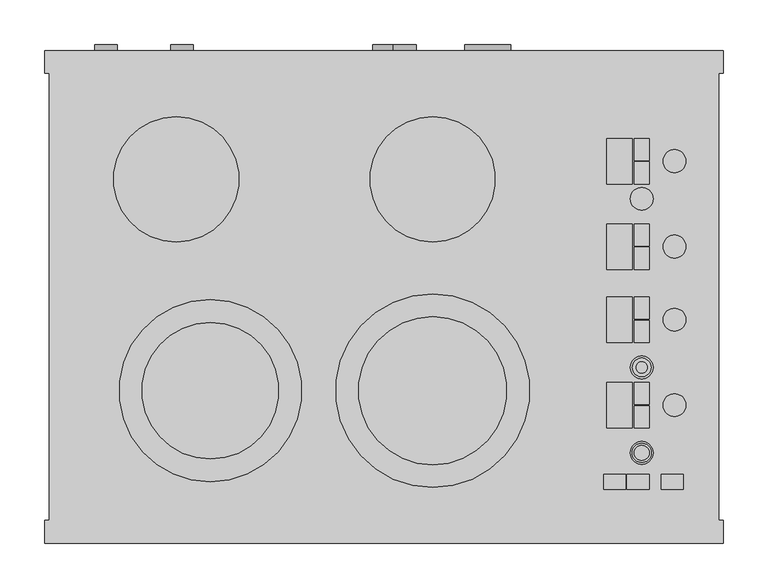
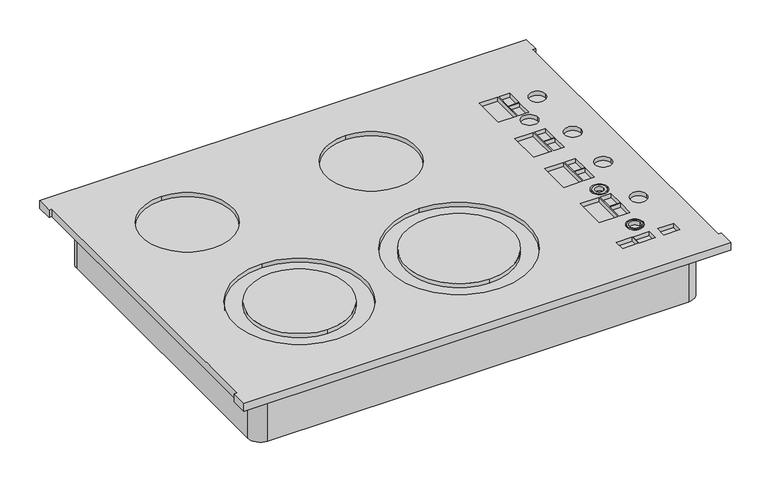
"""IFC4 building model written with IfcOpenShell, lengths in millimetres: proxy geometry, Cooktops_Electric_GE-Monogram_ZEU30RSFSS : Cooktops_Electric_GE-Monogram_ZEU30RSFSS."""

from ifc_helpers import new_model, si_unit, point, frame, frame_2d, origin, origin_with_axes, place, context, project, spatial, polyline, circle_curve, trimmed, segment, composite_curve, outline, extrude, source, transform, mapped, element, save


def specialty_equipment_065d487b(model_context):
    return source(origin(), model_context, "Body", "SweptSolid", [
        extrude(outline(composite_curve([segment(polyline([(-377.825, 274.6375), (377.825, 274.6375), (377.825, 249.2375), (373.215296, 249.2375), (373.215296, -249.2375), (377.825, -249.2375), (377.825, -274.6375)]), True, "CONTINUOUS"), segment(trimmed(circle_curve(frame_2d((0.0, 4104.744837)), 4395.65028), [point((377.825, -274.6375))], [point((-377.825, -274.6375))], False, "CARTESIAN"), True, "CONTINUOUS"), segment(polyline([(-377.825, -274.6375), (-377.825, -249.2375), (-373.215296, -249.2375), (-373.215296, 249.2375), (-377.825, 249.2375), (-377.825, 274.6375)]), True, "CONTINUOUS")], self_intersect=False), holes=[composite_curve([segment(trimmed(circle_curve(frame_2d((54.2006403, 131.1676685)), 69.85), [point((54.2006403, 201.0176685))], [point((54.2006403, 61.3176685))], True, "CARTESIAN"), True, "CONTINUOUS"), segment(trimmed(circle_curve(frame_2d((54.2006403, 131.1676685)), 69.85), [point((54.2006403, 61.3176685))], [point((54.2006403, 201.0176685))], True, "CARTESIAN"), True, "CONTINUOUS")], self_intersect=False), composite_curve([segment(trimmed(circle_curve(frame_2d((54.2006403, -104.6769785)), 107.95), [point((54.2006403, 3.2730215))], [point((54.2006403, -212.6269785))], True, "CARTESIAN"), True, "CONTINUOUS"), segment(trimmed(circle_curve(frame_2d((54.2006403, -104.6769785)), 107.95), [point((54.2006403, -212.6269785))], [point((54.2006403, 3.2730215))], True, "CARTESIAN"), True, "CONTINUOUS")], self_intersect=False), composite_curve([segment(trimmed(circle_curve(frame_2d((-193.4493597, -104.6769785)), 101.6), [point((-193.4493597, -3.0769785))], [point((-193.4493597, -206.2769785))], True, "CARTESIAN"), True, "CONTINUOUS"), segment(trimmed(circle_curve(frame_2d((-193.4493597, -104.6769785)), 101.6), [point((-193.4493597, -206.2769785))], [point((-193.4493597, -3.0769785))], True, "CARTESIAN"), True, "CONTINUOUS")], self_intersect=False), composite_curve([segment(trimmed(circle_curve(frame_2d((-231.5493597, 131.1676685)), 69.85), [point((-231.5493597, 201.0176685))], [point((-231.5493597, 61.3176685))], True, "CARTESIAN"), True, "CONTINUOUS"), segment(trimmed(circle_curve(frame_2d((-231.5493597, 131.1676685)), 69.85), [point((-231.5493597, 61.3176685))], [point((-231.5493597, 201.0176685))], True, "CARTESIAN"), True, "CONTINUOUS")], self_intersect=False), polyline([(276.5029806, 125.8458819), (276.5029806, 176.6458819), (247.9432042, 176.6458819), (247.9432042, 125.8458819), (276.5029806, 125.8458819)]), polyline([(295.3523984, 125.8458819), (295.3523984, 150.5447711), (278.8954782, 150.5447711), (278.8954782, 125.8458819), (295.3523984, 125.8458819)]), polyline([(295.3523984, 176.6458819), (278.8954782, 176.6458819), (278.8954782, 151.9469928), (295.3523984, 151.9469928), (295.3523984, 176.6458819)]), composite_curve([segment(trimmed(circle_curve(frame_2d((323.5654873, 151.2458819)), 12.7), [point((310.8654873, 151.2458819))], [point((336.2654873, 151.2458819))], True, "CARTESIAN"), True, "CONTINUOUS"), segment(trimmed(circle_curve(frame_2d((323.5654873, 151.2458819)), 12.7), [point((336.2654873, 151.2458819))], [point((310.8654873, 151.2458819))], True, "CARTESIAN"), True, "CONTINUOUS")], self_intersect=False), composite_curve([segment(trimmed(circle_curve(frame_2d((287.1239383, 109.3246752)), 12.7), [point((274.4239383, 109.3246752))], [point((299.8239383, 109.3246752))], True, "CARTESIAN"), True, "CONTINUOUS"), segment(trimmed(circle_curve(frame_2d((287.1239383, 109.3246752)), 12.7), [point((299.8239383, 109.3246752))], [point((274.4239383, 109.3246752))], True, "CARTESIAN"), True, "CONTINUOUS")], self_intersect=False), polyline([(276.5029806, 30.5958819), (276.5029806, 81.3958819), (247.9432042, 81.3958819), (247.9432042, 30.5958819), (276.5029806, 30.5958819)]), polyline([(295.3523984, 30.5958819), (295.3523984, 55.2947711), (278.8954782, 55.2947711), (278.8954782, 30.5958819), (295.3523984, 30.5958819)]), polyline([(295.3523984, 81.3958819), (278.8954782, 81.3958819), (278.8954782, 56.6969928), (295.3523984, 56.6969928), (295.3523984, 81.3958819)]), composite_curve([segment(trimmed(circle_curve(frame_2d((323.5654873, 55.9958819)), 12.7), [point((310.8654873, 55.9958819))], [point((336.2654873, 55.9958819))], True, "CARTESIAN"), True, "CONTINUOUS"), segment(trimmed(circle_curve(frame_2d((323.5654873, 55.9958819)), 12.7), [point((336.2654873, 55.9958819))], [point((310.8654873, 55.9958819))], True, "CARTESIAN"), True, "CONTINUOUS")], self_intersect=False), polyline([(276.5029806, -95.25), (247.9432042, -95.25), (247.9432042, -146.05), (276.5029806, -146.05), (276.5029806, -95.25)]), polyline([(295.3523984, -95.25), (278.8954782, -95.25), (278.8954782, -119.9488891), (295.3523984, -119.9488891), (295.3523984, -95.25)]), polyline([(295.3523984, -146.05), (295.3523984, -121.3511109), (278.8954782, -121.3511109), (278.8954782, -146.05), (295.3523984, -146.05)]), composite_curve([segment(trimmed(circle_curve(frame_2d((323.5654873, -120.65)), 12.7), [point((310.8654873, -120.65))], [point((336.2654873, -120.65))], True, "CARTESIAN"), True, "CONTINUOUS"), segment(trimmed(circle_curve(frame_2d((323.5654873, -120.65)), 12.7), [point((336.2654873, -120.65))], [point((310.8654873, -120.65))], True, "CARTESIAN"), True, "CONTINUOUS")], self_intersect=False), composite_curve([segment(trimmed(circle_curve(frame_2d((287.1239383, -78.7287933)), 12.7), [point((274.4239383, -78.7287933))], [point((299.8239383, -78.7287933))], True, "CARTESIAN"), True, "CONTINUOUS"), segment(trimmed(circle_curve(frame_2d((287.1239383, -78.7287933)), 12.7), [point((299.8239383, -78.7287933))], [point((274.4239383, -78.7287933))], True, "CARTESIAN"), True, "CONTINUOUS")], self_intersect=False), polyline([(276.5029806, 0.0), (247.9432042, 0.0), (247.9432042, -50.8), (276.5029806, -50.8), (276.5029806, 0.0)]), polyline([(295.3523984, 0.0), (278.8954782, 0.0), (278.8954782, -24.6988891), (295.3523984, -24.6988891), (295.3523984, 0.0)]), polyline([(295.3523984, -50.8), (295.3523984, -26.1011109), (278.8954782, -26.1011109), (278.8954782, -50.8), (295.3523984, -50.8)]), composite_curve([segment(trimmed(circle_curve(frame_2d((323.5654873, -25.4)), 12.7), [point((310.8654873, -25.4))], [point((336.2654873, -25.4))], True, "CARTESIAN"), True, "CONTINUOUS"), segment(trimmed(circle_curve(frame_2d((323.5654873, -25.4)), 12.7), [point((336.2654873, -25.4))], [point((310.8654873, -25.4))], True, "CARTESIAN"), True, "CONTINUOUS")], self_intersect=False), composite_curve([segment(trimmed(circle_curve(frame_2d((287.1239383, -173.9787933)), 12.7), [point((274.4239383, -173.9787933))], [point((299.8239383, -173.9787933))], True, "CARTESIAN"), True, "CONTINUOUS"), segment(trimmed(circle_curve(frame_2d((287.1239383, -173.9787933)), 12.7), [point((299.8239383, -173.9787933))], [point((274.4239383, -173.9787933))], True, "CARTESIAN"), True, "CONTINUOUS")], self_intersect=False), polyline([(295.3523984, -214.5130009), (295.3523984, -198.0560807), (270.6535092, -198.0560807), (270.6535092, -214.5130009), (295.3523984, -214.5130009)]), polyline([(244.5523984, -214.5130009), (269.2512875, -214.5130009), (269.2512875, -198.0560807), (244.5523984, -198.0560807), (244.5523984, -214.5130009)]), polyline([(333.4523984, -214.5130009), (333.4523984, -198.0560807), (308.7535092, -198.0560807), (308.7535092, -214.5130009), (333.4523984, -214.5130009)])]), frame((0.0, 0.0, 82.55), z_axis=(0.0, 0.0, 1.0), x_axis=(1.0, 0.0, 0.0)), (0.0, 0.0, 1.0), 12.7),
        extrude(outline(composite_curve([segment(trimmed(circle_curve(frame_2d((54.2006403, -104.6769785)), 82.55), [point((54.2006403, -22.1269785))], [point((54.2006403, -187.2269785))], False, "CARTESIAN"), True, "CONTINUOUS"), segment(trimmed(circle_curve(frame_2d((54.2006403, -104.6769785)), 82.55), [point((54.2006403, -187.2269785))], [point((54.2006403, -22.1269785))], False, "CARTESIAN"), True, "CONTINUOUS")], self_intersect=False)), frame((0.0, 0.0, 82.55), z_axis=(0.0, 0.0, 1.0), x_axis=(1.0, 0.0, 0.0)), (0.0, 0.0, 1.0), 12.7),
        extrude(outline(composite_curve([segment(trimmed(circle_curve(frame_2d((-193.4493597, -104.6769785)), 76.2), [point((-193.4493597, -28.4769785))], [point((-193.4493597, -180.8769785))], False, "CARTESIAN"), True, "CONTINUOUS"), segment(trimmed(circle_curve(frame_2d((-193.4493597, -104.6769785)), 76.2), [point((-193.4493597, -180.8769785))], [point((-193.4493597, -28.4769785))], False, "CARTESIAN"), True, "CONTINUOUS")], self_intersect=False)), frame((0.0, 0.0, 82.55), z_axis=(0.0, 0.0, 1.0), x_axis=(1.0, 0.0, 0.0)), (0.0, 0.0, 1.0), 12.7),
        extrude(outline(composite_curve([segment(trimmed(circle_curve(frame_2d((287.1239383, -173.9787933)), 10.7837612), [point((276.3401772, -173.9787933))], [point((297.9076995, -173.9787933))], False, "CARTESIAN"), True, "CONTINUOUS"), segment(trimmed(circle_curve(frame_2d((287.1239383, -173.9787933)), 10.7837612), [point((297.9076995, -173.9787933))], [point((276.3401772, -173.9787933))], False, "CARTESIAN"), True, "CONTINUOUS")], self_intersect=False), holes=[composite_curve([segment(trimmed(circle_curve(frame_2d((287.1239383, -173.9787933)), 8.3684562), [point((278.7554821, -173.9787933))], [point((295.4923945, -173.9787933))], True, "CARTESIAN"), True, "CONTINUOUS"), segment(trimmed(circle_curve(frame_2d((287.1239383, -173.9787933)), 8.3684562), [point((295.4923945, -173.9787933))], [point((278.7554821, -173.9787933))], True, "CARTESIAN"), True, "CONTINUOUS")], self_intersect=False)]), frame((0.0, 0.0, 82.55), z_axis=(0.0, 0.0, 1.0), x_axis=(1.0, 0.0, 0.0)), (0.0, 0.0, 1.0), 12.7),
        extrude(outline(composite_curve([segment(trimmed(circle_curve(frame_2d((287.1239383, -78.7287933)), 10.3621749), [point((276.7617634, -78.7287933))], [point((297.4861132, -78.7287933))], False, "CARTESIAN"), True, "CONTINUOUS"), segment(trimmed(circle_curve(frame_2d((287.1239383, -78.7287933)), 10.3621749), [point((297.4861132, -78.7287933))], [point((276.7617634, -78.7287933))], False, "CARTESIAN"), True, "CONTINUOUS")], self_intersect=False), holes=[composite_curve([segment(trimmed(circle_curve(frame_2d((287.1239383, -78.7287933)), 6.35), [point((280.7739383, -78.7287933))], [point((293.4739383, -78.7287933))], True, "CARTESIAN"), True, "CONTINUOUS"), segment(trimmed(circle_curve(frame_2d((287.1239383, -78.7287933)), 6.35), [point((293.4739383, -78.7287933))], [point((280.7739383, -78.7287933))], True, "CARTESIAN"), True, "CONTINUOUS")], self_intersect=False)]), frame((0.0, 0.0, 82.55), z_axis=(0.0, 0.0, 1.0), x_axis=(1.0, 0.0, 0.0)), (0.0, 0.0, 1.0), 12.7),
        extrude(outline(polyline([(276.5029806, 125.8458819), (247.9432042, 125.8458819), (247.9432042, 176.6458819), (276.5029806, 176.6458819), (276.5029806, 125.8458819)])), frame((0.0, 0.0, 82.55), z_axis=(0.0, 0.0, 1.0), x_axis=(1.0, 0.0, 0.0)), (0.0, 0.0, 1.0), 6.35),
        extrude(outline(polyline([(295.3523984, 125.8458819), (278.8954782, 125.8458819), (278.8954782, 150.5447711), (295.3523984, 150.5447711), (295.3523984, 125.8458819)])), frame((0.0, 0.0, 82.55), z_axis=(0.0, 0.0, 1.0), x_axis=(1.0, 0.0, 0.0)), (0.0, 0.0, 1.0), 6.35),
        extrude(outline(polyline([(295.3523984, 176.6458819), (295.3523984, 151.9469928), (278.8954782, 151.9469928), (278.8954782, 176.6458819), (295.3523984, 176.6458819)])), frame((0.0, 0.0, 82.55), z_axis=(0.0, 0.0, 1.0), x_axis=(1.0, 0.0, 0.0)), (0.0, 0.0, 1.0), 6.35),
        extrude(outline(composite_curve([segment(trimmed(circle_curve(frame_2d((323.5654873, 151.2458819)), 12.7), [point((310.8654873, 151.2458819))], [point((336.2654873, 151.2458819))], False, "CARTESIAN"), True, "CONTINUOUS"), segment(trimmed(circle_curve(frame_2d((323.5654873, 151.2458819)), 12.7), [point((336.2654873, 151.2458819))], [point((310.8654873, 151.2458819))], False, "CARTESIAN"), True, "CONTINUOUS")], self_intersect=False)), frame((0.0, 0.0, 82.55), z_axis=(0.0, 0.0, 1.0), x_axis=(1.0, 0.0, 0.0)), (0.0, 0.0, 1.0), 6.35),
        extrude(outline(composite_curve([segment(trimmed(circle_curve(frame_2d((287.1239383, 109.3246752)), 12.7), [point((274.4239383, 109.3246752))], [point((299.8239383, 109.3246752))], False, "CARTESIAN"), True, "CONTINUOUS"), segment(trimmed(circle_curve(frame_2d((287.1239383, 109.3246752)), 12.7), [point((299.8239383, 109.3246752))], [point((274.4239383, 109.3246752))], False, "CARTESIAN"), True, "CONTINUOUS")], self_intersect=False)), frame((0.0, 0.0, 82.55), z_axis=(0.0, 0.0, 1.0), x_axis=(1.0, 0.0, 0.0)), (0.0, 0.0, 1.0), 6.35),
        extrude(outline(polyline([(276.5029806, 30.5958819), (247.9432042, 30.5958819), (247.9432042, 81.3958819), (276.5029806, 81.3958819), (276.5029806, 30.5958819)])), frame((0.0, 0.0, 82.55), z_axis=(0.0, 0.0, 1.0), x_axis=(1.0, 0.0, 0.0)), (0.0, 0.0, 1.0), 6.35),
        extrude(outline(polyline([(295.3523984, 30.5958819), (278.8954782, 30.5958819), (278.8954782, 55.2947711), (295.3523984, 55.2947711), (295.3523984, 30.5958819)])), frame((0.0, 0.0, 82.55), z_axis=(0.0, 0.0, 1.0), x_axis=(1.0, 0.0, 0.0)), (0.0, 0.0, 1.0), 6.35),
        extrude(outline(polyline([(295.3523984, 81.3958819), (295.3523984, 56.6969928), (278.8954782, 56.6969928), (278.8954782, 81.3958819), (295.3523984, 81.3958819)])), frame((0.0, 0.0, 82.55), z_axis=(0.0, 0.0, 1.0), x_axis=(1.0, 0.0, 0.0)), (0.0, 0.0, 1.0), 6.35),
        extrude(outline(composite_curve([segment(trimmed(circle_curve(frame_2d((323.5654873, 55.9958819)), 12.7), [point((310.8654873, 55.9958819))], [point((336.2654873, 55.9958819))], False, "CARTESIAN"), True, "CONTINUOUS"), segment(trimmed(circle_curve(frame_2d((323.5654873, 55.9958819)), 12.7), [point((336.2654873, 55.9958819))], [point((310.8654873, 55.9958819))], False, "CARTESIAN"), True, "CONTINUOUS")], self_intersect=False)), frame((0.0, 0.0, 82.55), z_axis=(0.0, 0.0, 1.0), x_axis=(1.0, 0.0, 0.0)), (0.0, 0.0, 1.0), 6.35),
        extrude(outline(polyline([(276.5029806, -95.25), (276.5029806, -146.05), (247.9432042, -146.05), (247.9432042, -95.25), (276.5029806, -95.25)])), frame((0.0, 0.0, 82.55), z_axis=(0.0, 0.0, 1.0), x_axis=(1.0, 0.0, 0.0)), (0.0, 0.0, 1.0), 6.35),
        extrude(outline(polyline([(295.3523984, -95.25), (295.3523984, -119.9488891), (278.8954782, -119.9488891), (278.8954782, -95.25), (295.3523984, -95.25)])), frame((0.0, 0.0, 82.55), z_axis=(0.0, 0.0, 1.0), x_axis=(1.0, 0.0, 0.0)), (0.0, 0.0, 1.0), 6.35),
        extrude(outline(polyline([(295.3523984, -146.05), (278.8954782, -146.05), (278.8954782, -121.3511109), (295.3523984, -121.3511109), (295.3523984, -146.05)])), frame((0.0, 0.0, 82.55), z_axis=(0.0, 0.0, 1.0), x_axis=(1.0, 0.0, 0.0)), (0.0, 0.0, 1.0), 6.35),
        extrude(outline(composite_curve([segment(trimmed(circle_curve(frame_2d((323.5654873, -120.65)), 12.7), [point((310.8654873, -120.65))], [point((336.2654873, -120.65))], False, "CARTESIAN"), True, "CONTINUOUS"), segment(trimmed(circle_curve(frame_2d((323.5654873, -120.65)), 12.7), [point((336.2654873, -120.65))], [point((310.8654873, -120.65))], False, "CARTESIAN"), True, "CONTINUOUS")], self_intersect=False)), frame((0.0, 0.0, 82.55), z_axis=(0.0, 0.0, 1.0), x_axis=(1.0, 0.0, 0.0)), (0.0, 0.0, 1.0), 6.35),
        extrude(outline(composite_curve([segment(trimmed(circle_curve(frame_2d((287.1239383, -78.7287933)), 12.7), [point((274.4239383, -78.7287933))], [point((299.8239383, -78.7287933))], False, "CARTESIAN"), True, "CONTINUOUS"), segment(trimmed(circle_curve(frame_2d((287.1239383, -78.7287933)), 12.7), [point((299.8239383, -78.7287933))], [point((274.4239383, -78.7287933))], False, "CARTESIAN"), True, "CONTINUOUS")], self_intersect=False), holes=[composite_curve([segment(trimmed(circle_curve(frame_2d((287.1239383, -78.7287933)), 10.3621749), [point((276.7617634, -78.7287933))], [point((297.4861132, -78.7287933))], True, "CARTESIAN"), True, "CONTINUOUS"), segment(trimmed(circle_curve(frame_2d((287.1239383, -78.7287933)), 10.3621749), [point((297.4861132, -78.7287933))], [point((276.7617634, -78.7287933))], True, "CARTESIAN"), True, "CONTINUOUS")], self_intersect=False)]), frame((0.0, 0.0, 82.55), z_axis=(0.0, 0.0, 1.0), x_axis=(1.0, 0.0, 0.0)), (0.0, 0.0, 1.0), 6.35),
        extrude(outline(polyline([(276.5029806, 0.0), (276.5029806, -50.8), (247.9432042, -50.8), (247.9432042, 0.0), (276.5029806, 0.0)])), frame((0.0, 0.0, 82.55), z_axis=(0.0, 0.0, 1.0), x_axis=(1.0, 0.0, 0.0)), (0.0, 0.0, 1.0), 6.35),
        extrude(outline(polyline([(295.3523984, 0.0), (295.3523984, -24.6988891), (278.8954782, -24.6988891), (278.8954782, 0.0), (295.3523984, 0.0)])), frame((0.0, 0.0, 82.55), z_axis=(0.0, 0.0, 1.0), x_axis=(1.0, 0.0, 0.0)), (0.0, 0.0, 1.0), 6.35),
        extrude(outline(polyline([(295.3523984, -50.8), (278.8954782, -50.8), (278.8954782, -26.1011109), (295.3523984, -26.1011109), (295.3523984, -50.8)])), frame((0.0, 0.0, 82.55), z_axis=(0.0, 0.0, 1.0), x_axis=(1.0, 0.0, 0.0)), (0.0, 0.0, 1.0), 6.35),
        extrude(outline(composite_curve([segment(trimmed(circle_curve(frame_2d((323.5654873, -25.4)), 12.7), [point((310.8654873, -25.4))], [point((336.2654873, -25.4))], False, "CARTESIAN"), True, "CONTINUOUS"), segment(trimmed(circle_curve(frame_2d((323.5654873, -25.4)), 12.7), [point((336.2654873, -25.4))], [point((310.8654873, -25.4))], False, "CARTESIAN"), True, "CONTINUOUS")], self_intersect=False)), frame((0.0, 0.0, 82.55), z_axis=(0.0, 0.0, 1.0), x_axis=(1.0, 0.0, 0.0)), (0.0, 0.0, 1.0), 6.35),
        extrude(outline(composite_curve([segment(trimmed(circle_curve(frame_2d((287.1239383, -173.9787933)), 12.7), [point((274.4239383, -173.9787933))], [point((299.8239383, -173.9787933))], False, "CARTESIAN"), True, "CONTINUOUS"), segment(trimmed(circle_curve(frame_2d((287.1239383, -173.9787933)), 12.7), [point((299.8239383, -173.9787933))], [point((274.4239383, -173.9787933))], False, "CARTESIAN"), True, "CONTINUOUS")], self_intersect=False), holes=[composite_curve([segment(trimmed(circle_curve(frame_2d((287.1239383, -173.9787933)), 10.7837612), [point((276.3401772, -173.9787933))], [point((297.9076995, -173.9787933))], True, "CARTESIAN"), True, "CONTINUOUS"), segment(trimmed(circle_curve(frame_2d((287.1239383, -173.9787933)), 10.7837612), [point((297.9076995, -173.9787933))], [point((276.3401772, -173.9787933))], True, "CARTESIAN"), True, "CONTINUOUS")], self_intersect=False)]), frame((0.0, 0.0, 82.55), z_axis=(0.0, 0.0, 1.0), x_axis=(1.0, 0.0, 0.0)), (0.0, 0.0, 1.0), 6.35),
        extrude(outline(composite_curve([segment(trimmed(circle_curve(frame_2d((287.1239383, -173.9787933)), 8.3684562), [point((278.7554821, -173.9787933))], [point((295.4923945, -173.9787933))], False, "CARTESIAN"), True, "CONTINUOUS"), segment(trimmed(circle_curve(frame_2d((287.1239383, -173.9787933)), 8.3684562), [point((295.4923945, -173.9787933))], [point((278.7554821, -173.9787933))], False, "CARTESIAN"), True, "CONTINUOUS")], self_intersect=False)), frame((0.0, 0.0, 82.55), z_axis=(0.0, 0.0, 1.0), x_axis=(1.0, 0.0, 0.0)), (0.0, 0.0, 1.0), 6.35),
        extrude(outline(composite_curve([segment(trimmed(circle_curve(frame_2d((287.1239383, -78.7287933)), 6.35), [point((280.7739383, -78.7287933))], [point((293.4739383, -78.7287933))], False, "CARTESIAN"), True, "CONTINUOUS"), segment(trimmed(circle_curve(frame_2d((287.1239383, -78.7287933)), 6.35), [point((293.4739383, -78.7287933))], [point((280.7739383, -78.7287933))], False, "CARTESIAN"), True, "CONTINUOUS")], self_intersect=False)), frame((0.0, 0.0, 82.55), z_axis=(0.0, 0.0, 1.0), x_axis=(1.0, 0.0, 0.0)), (0.0, 0.0, 1.0), 6.35),
        extrude(outline(polyline([(295.3523984, -214.5130009), (270.6535092, -214.5130009), (270.6535092, -198.0560807), (295.3523984, -198.0560807), (295.3523984, -214.5130009)])), frame((0.0, 0.0, 82.55), z_axis=(0.0, 0.0, 1.0), x_axis=(1.0, 0.0, 0.0)), (0.0, 0.0, 1.0), 6.35),
        extrude(outline(polyline([(244.5523984, -214.5130009), (244.5523984, -198.0560807), (269.2512875, -198.0560807), (269.2512875, -214.5130009), (244.5523984, -214.5130009)])), frame((0.0, 0.0, 82.55), z_axis=(0.0, 0.0, 1.0), x_axis=(1.0, 0.0, 0.0)), (0.0, 0.0, 1.0), 6.35),
        extrude(outline(polyline([(333.4523984, -214.5130009), (308.7535092, -214.5130009), (308.7535092, -198.0560807), (333.4523984, -198.0560807), (333.4523984, -214.5130009)])), frame((0.0, 0.0, 82.55), z_axis=(0.0, 0.0, 1.0), x_axis=(1.0, 0.0, 0.0)), (0.0, 0.0, 1.0), 6.35),
        extrude(outline(composite_curve([segment(trimmed(circle_curve(frame_2d((54.2006403, 131.1676685)), 69.85), [point((54.2006403, 201.0176685))], [point((54.2006403, 61.3176685))], False, "CARTESIAN"), True, "CONTINUOUS"), segment(trimmed(circle_curve(frame_2d((54.2006403, 131.1676685)), 69.85), [point((54.2006403, 61.3176685))], [point((54.2006403, 201.0176685))], False, "CARTESIAN"), True, "CONTINUOUS")], self_intersect=False)), frame((0.0, 0.0, 82.55), z_axis=(0.0, 0.0, 1.0), x_axis=(1.0, 0.0, 0.0)), (0.0, 0.0, 1.0), 6.35),
        extrude(outline(composite_curve([segment(trimmed(circle_curve(frame_2d((54.2006403, -104.6769785)), 107.95), [point((54.2006403, 3.2730215))], [point((54.2006403, -212.6269785))], False, "CARTESIAN"), True, "CONTINUOUS"), segment(trimmed(circle_curve(frame_2d((54.2006403, -104.6769785)), 107.95), [point((54.2006403, -212.6269785))], [point((54.2006403, 3.2730215))], False, "CARTESIAN"), True, "CONTINUOUS")], self_intersect=False), holes=[composite_curve([segment(trimmed(circle_curve(frame_2d((54.2006403, -104.6769785)), 82.55), [point((54.2006403, -22.1269785))], [point((54.2006403, -187.2269785))], True, "CARTESIAN"), True, "CONTINUOUS"), segment(trimmed(circle_curve(frame_2d((54.2006403, -104.6769785)), 82.55), [point((54.2006403, -187.2269785))], [point((54.2006403, -22.1269785))], True, "CARTESIAN"), True, "CONTINUOUS")], self_intersect=False)]), frame((0.0, 0.0, 82.55), z_axis=(0.0, 0.0, 1.0), x_axis=(1.0, 0.0, 0.0)), (0.0, 0.0, 1.0), 6.35),
        extrude(outline(composite_curve([segment(trimmed(circle_curve(frame_2d((-193.4493597, -104.6769785)), 101.6), [point((-193.4493597, -3.0769785))], [point((-193.4493597, -206.2769785))], False, "CARTESIAN"), True, "CONTINUOUS"), segment(trimmed(circle_curve(frame_2d((-193.4493597, -104.6769785)), 101.6), [point((-193.4493597, -206.2769785))], [point((-193.4493597, -3.0769785))], False, "CARTESIAN"), True, "CONTINUOUS")], self_intersect=False), holes=[composite_curve([segment(trimmed(circle_curve(frame_2d((-193.4493597, -104.6769785)), 76.2), [point((-193.4493597, -28.4769785))], [point((-193.4493597, -180.8769785))], True, "CARTESIAN"), True, "CONTINUOUS"), segment(trimmed(circle_curve(frame_2d((-193.4493597, -104.6769785)), 76.2), [point((-193.4493597, -180.8769785))], [point((-193.4493597, -28.4769785))], True, "CARTESIAN"), True, "CONTINUOUS")], self_intersect=False)]), frame((0.0, 0.0, 82.55), z_axis=(0.0, 0.0, 1.0), x_axis=(1.0, 0.0, 0.0)), (0.0, 0.0, 1.0), 6.35),
        extrude(outline(composite_curve([segment(trimmed(circle_curve(frame_2d((-231.5493597, 131.1676685)), 69.85), [point((-231.5493597, 201.0176685))], [point((-231.5493597, 61.3176685))], False, "CARTESIAN"), True, "CONTINUOUS"), segment(trimmed(circle_curve(frame_2d((-231.5493597, 131.1676685)), 69.85), [point((-231.5493597, 61.3176685))], [point((-231.5493597, 201.0176685))], False, "CARTESIAN"), True, "CONTINUOUS")], self_intersect=False)), frame((0.0, 0.0, 82.55), z_axis=(0.0, 0.0, 1.0), x_axis=(1.0, 0.0, 0.0)), (0.0, 0.0, 1.0), 6.35),
        extrude(outline(composite_curve([segment(trimmed(circle_curve(frame_2d((44.45, 0.0)), 12.7), [point((44.45, 12.7))], [point((44.45, -12.7))], False, "CARTESIAN"), True, "CONTINUOUS"), segment(trimmed(circle_curve(frame_2d((44.45, 0.0)), 12.7), [point((44.45, -12.7))], [point((44.45, 12.7))], False, "CARTESIAN"), True, "CONTINUOUS")], self_intersect=False)), frame((0.0, 274.6375, 0.0), z_axis=(0.0, 1.0, 0.0), x_axis=(0.0, 0.0, 1.0)), (0.0, 0.0, 1.0), 6.35),
        extrude(outline(composite_curve([segment(trimmed(circle_curve(frame_2d((48.3374744, -309.8039599)), 12.7), [point((48.3374744, -297.1039599))], [point((48.3374744, -322.5039599))], False, "CARTESIAN"), True, "CONTINUOUS"), segment(trimmed(circle_curve(frame_2d((48.3374744, -309.8039599)), 12.7), [point((48.3374744, -322.5039599))], [point((48.3374744, -297.1039599))], False, "CARTESIAN"), True, "CONTINUOUS")], self_intersect=False)), frame((0.0, 274.6375, 0.0), z_axis=(0.0, 1.0, 0.0), x_axis=(0.0, 0.0, 1.0)), (0.0, 0.0, 1.0), 6.35),
        extrude(outline(composite_curve([segment(trimmed(circle_curve(frame_2d((45.2599524, -225.0070053)), 12.7), [point((45.2599524, -212.3070053))], [point((45.2599524, -237.7070053))], False, "CARTESIAN"), True, "CONTINUOUS"), segment(trimmed(circle_curve(frame_2d((45.2599524, -225.0070053)), 12.7), [point((45.2599524, -237.7070053))], [point((45.2599524, -212.3070053))], False, "CARTESIAN"), True, "CONTINUOUS")], self_intersect=False)), frame((0.0, 274.6375, 0.0), z_axis=(0.0, 1.0, 0.0), x_axis=(0.0, 0.0, 1.0)), (0.0, 0.0, 1.0), 6.35),
        extrude(outline(composite_curve([segment(trimmed(circle_curve(frame_2d((72.9920745, 23.2492285)), 12.7), [point((72.9920745, 35.9492285))], [point((72.9920745, 10.5492285))], False, "CARTESIAN"), True, "CONTINUOUS"), segment(trimmed(circle_curve(frame_2d((72.9920745, 23.2492285)), 12.7), [point((72.9920745, 10.5492285))], [point((72.9920745, 35.9492285))], False, "CARTESIAN"), True, "CONTINUOUS")], self_intersect=False)), frame((0.0, 274.6375, 0.0), z_axis=(0.0, 1.0, 0.0), x_axis=(0.0, 0.0, 1.0)), (0.0, 0.0, 1.0), 6.35),
        extrude(outline(composite_curve([segment(polyline([(-346.075, -230.1875), (-346.075, 230.1875)]), True, "CONTINUOUS"), segment(trimmed(circle_curve(frame_2d((-327.025, 230.1875)), 19.05), [point((-346.075, 230.1875))], [point((-327.025, 249.2375))], False, "CARTESIAN"), True, "CONTINUOUS"), segment(polyline([(-327.025, 249.2375), (327.025, 249.2375)]), True, "CONTINUOUS"), segment(trimmed(circle_curve(frame_2d((327.025, 230.1875)), 19.05), [point((327.025, 249.2375))], [point((346.075, 230.1875))], False, "CARTESIAN"), True, "CONTINUOUS"), segment(polyline([(346.075, 230.1875), (346.075, -230.1875)]), True, "CONTINUOUS"), segment(trimmed(circle_curve(frame_2d((327.025, -230.1875)), 19.05), [point((346.075, -230.1875))], [point((327.025, -249.2375))], False, "CARTESIAN"), True, "CONTINUOUS"), segment(polyline([(327.025, -249.2375), (-327.025, -249.2375)]), True, "CONTINUOUS"), segment(trimmed(circle_curve(frame_2d((-327.025, -230.1875)), 19.05), [point((-327.025, -249.2375))], [point((-346.075, -230.1875))], False, "CARTESIAN"), True, "CONTINUOUS")], self_intersect=False), holes=[composite_curve([segment(polyline([(333.375, -230.1875), (333.375, 230.1875)]), True, "CONTINUOUS"), segment(trimmed(circle_curve(frame_2d((327.025, 230.1875)), 6.35), [point((333.375, 230.1875))], [point((327.025, 236.5375))], True, "CARTESIAN"), True, "CONTINUOUS"), segment(polyline([(327.025, 236.5375), (-327.025, 236.5375)]), True, "CONTINUOUS"), segment(trimmed(circle_curve(frame_2d((-327.025, 230.1875)), 6.35), [point((-327.025, 236.5375))], [point((-333.375, 230.1875))], True, "CARTESIAN"), True, "CONTINUOUS"), segment(polyline([(-333.375, 230.1875), (-333.375, -230.1875)]), True, "CONTINUOUS"), segment(trimmed(circle_curve(frame_2d((-327.025, -230.1875)), 6.35), [point((-333.375, -230.1875))], [point((-327.025, -236.5375))], True, "CARTESIAN"), True, "CONTINUOUS"), segment(polyline([(-327.025, -236.5375), (327.025, -236.5375)]), True, "CONTINUOUS"), segment(trimmed(circle_curve(frame_2d((327.025, -230.1875)), 6.35), [point((327.025, -236.5375))], [point((333.375, -230.1875))], True, "CARTESIAN"), True, "CONTINUOUS")], self_intersect=False)]), origin_with_axes(), (0.0, 0.0, 1.0), 82.55),
        extrude(outline(composite_curve([segment(trimmed(circle_curve(frame_2d((45.4406193, 115.6172129)), 25.4), [point((45.4406193, 141.0172129))], [point((45.4406193, 90.2172129))], False, "CARTESIAN"), True, "CONTINUOUS"), segment(trimmed(circle_curve(frame_2d((45.4406193, 115.6172129)), 25.4), [point((45.4406193, 90.2172129))], [point((45.4406193, 141.0172129))], False, "CARTESIAN"), True, "CONTINUOUS")], self_intersect=False)), frame((0.0, 274.6375, 0.0), z_axis=(0.0, 1.0, 0.0), x_axis=(0.0, 0.0, 1.0)), (0.0, 0.0, 1.0), 6.35),
    ])


if __name__ == "__main__":
    model = new_model("IFC4")
    model_context = context("Model", 3, world=origin())
    ifc_project = project(units=[si_unit("LENGTHUNIT", "METRE", prefix="MILLI")], contexts=[model_context])
    site = spatial("IfcSite", under=ifc_project)
    building = spatial("IfcBuilding", under=site)
    placement = place(None, origin())
    specialty_equipment_shape = specialty_equipment_065d487b(model_context)
    element("IfcBuildingElementProxy", 1, Name="Cooktops_Electric_GE-Monogram_ZEU30RSFSS : Cooktops_Electric_GE-Monogram_ZEU30RSFSS", ObjectType="Cooktops_Electric_GE-Monogram_ZEU30RSFSS : Cooktops_Electric_GE-Monogram_ZEU30RSFSS", at=placement, inside=building, context=model_context, shape_type="MappedRepresentation", body=[
        mapped(specialty_equipment_shape, transform((0.0, 0.0, 0.0), x_axis=(1.0, 0.0, 0.0), y_axis=(0.0, 1.0, 0.0), z_axis=(0.0, 0.0, 1.0))),
    ])
    save(model, "model.ifc")

# Revit data of these elements
# Project information
#   Organization Name = "North Hills Home"
#   Building Name = "Barton Keep B&B"
#   COBie.CreatedBy = "design@eagle.com"
#   COBie.CreatedOn = "2016-10-27T05:31:11"
#   COBie.Facility.Name = "Barton Keep B&B"
#   COBie.Facility.Category = "11-16 11 17:Multiple Bedroom Family Residence"
#   COBie.Facility.ProjectName = "Barton Keep B&B"
#   COBie.Facility.LinearUnits = "Feet"
#   COBie.Facility.AreaUnits = "Square Feet"
#   COBie.Facility.VolumeUnits = "Cubic Feet"
#   COBie.Facility.CurrencyUnit = "Dollar"
#   COBie.Facility.AreaMeasurement = "Revit Default Area Calculation Method"
#   COBie.Facility.Phase = "Operations"
#   Classification.Facility.Description = "Multiple Bedroom Family Residence"
#   Classification.Facility.Number = "11-16 11 17"
#   Project Issue Date = "5/27/2003"
#   Project Status = "Complete"
#   Client Name = "Eagale Noth America"
#   Project Address = "1002 East Swedesford Road King of Prussia, PA 19406 United States"
#   Project Name = "Barton Keep B&B"
#   Project Number = "Project Number"
# Type "Cooktops_Electric_GE-Monogram_ZEU30RSFSS : Cooktops_Electric_GE-Monogram_ZEU30RSFSS"
#   COBie.Type.CreatedBy = "design@eagle.com"
#   COBie.Type.CreatedOn = "2016-10-27T05:31:12"
#   COBie.Type.Name = "Cooktops_Electric_GE-Monogram_ZEU30RSFSS_Cooktops_Electric_GE-Monogram_ZEU30RSFSS"
#   COBie.Type.Category = "23-40 40 14 17 11 : Cookers, Ovens, Stoves"
#   COBie.Type.Description = "Cooktops_Electric_GE-Monogram_ZEU30RSFSS_Cooktops_Electric_GE-Monogram_ZEU30RSFSS"
#   COBie.Type.Manufacturer = "info@geappliances.com"
#   COBie.Type.ModelNumber = "As Specified in 11 30 00"
#   URL = "http://www.geappliances.com/"
#   Test Data = "http://www.geappliances.com/service_and_support/search.htm"
#   Specification = "http://www.arcat.com/sdspecs/htm/11450gea.htm"
#   SpecWizard = "http://www.arcat.com/specwizard/11450gea/index.htm?mf=&coid=32703"
#   Send Message = "http://www.arcat.com/users.pl?action=UserEmail&company=GE%20Appliances&coid=32703&rep=114&fax=502-452-0620&mf="
#   Sales Information = "http://www.geappliances.com/buy/"
#   Revision = "R1_02-2011"
#   Product Properties = "http://www.arcat.com/bim/bim_info.pl?fn=GEAppliances"
#   Product Data = "http://www.arcat.com/arcatcos/cos32/arc32703.html"
#   Model = "As Specified in 11 30 00"
#   Manufacturer Website = "http://www.geappliances.com/"
#   Manufacturer Phone - Toll Free = "800-626-2000"
#   Manufacturer Phone = "502-452-3346"
#   Manufacturer Fax = "502-452-0620"
#   Manufacturer Address = "Appliance Park AP4-109, Louisville, KY 40225"
#   Manufacturer = "info@geappliances.com"
#   Keynote = "11 30 00"
#   Installation-Fabrication = "http://www.geappliances.com/service_and_support/literature/"
#   Installation Phase = ""
#   Green Building-LEED = "http://www.geappliances.com/energy-star-appliances/"
#   Drawn By = "Sumex Design, Inc. / Robert S. Weygant, CSI, CDT, SCIP"
#   Description = "Residential Appliance as Specified in 11 30 00"
#   Copyright = "©Arcat Inc."
#   Construction Details = "http://www.geappliances.com/design_center/"
#   Building Codes = "http://www.geappliances.com/service_and_support/search.htm"
#   Assembly Code = "E1090400"
#   COBie.Type.ReplacementCost = 0
#   offset [instance default] = 0' - 0"
#   Voltage_MEP = 120 V
#   Unit Width = 2' - 5 3/4"
#   Unit Height = 0' - 3 1/4"
#   Unit Depth = 1' - 9 5/8"
#   MEP Apparent Power = 60 VA
#   MEP Amperage = 0.5 A
#   HWRad = 0' - 0 1/4"
#   GasRad = 0' - 0 1/4"
#   DrainRad = 0' - 0 5/8"
#   Connection Dia HW = 0' - 0 1/2"
#   Connection Dia Gas = 0' - 0 1/2"
#   Connection Dia DWV = 0' - 1 1/4"
#   Connection Dia CW = 0' - 0 1/2"
#   CWRad = 0' - 0 1/4"
#   COBie.Type = yes
#   Warranty Duration (Years) = 0
#   Maintenance Schedule (Months) = 0
#   Expected Lifespan (Years) = 0
#   Exterior Finish = ARCAT - Airspace
# Element 1 (IfcBuildingElementProxy, "Cooktops_Electric_GE-Monogram_ZEU30RSFSS : Cooktops_Electric_GE-Monogram_ZEU30RSFSS")
#   Materials on its faces: "ARCAT - Airspace", "Connector", "Gas", "Hot", "Cold", "Sanitary"
# Materials
#   "ARCAT - Airspace": class "Unassigned", colour RGB 255 255 255, transparency 0, Comments = "Rendering appearance not upgraded ", Description = "Air Space"
#   "Connector": class "Miscellaneous", colour RGB 255 255 0, transparency 0
#   "Gas": class "Miscellaneous", colour RGB 255 0 255, transparency 0
#   "Hot": class "Miscellaneous", colour RGB 255 0 0, transparency 0
#   "Cold": class "Miscellaneous", colour RGB 0 0 255, transparency 0
#   "Sanitary": class "Miscellaneous", colour RGB 0 255 0, transparency 0
